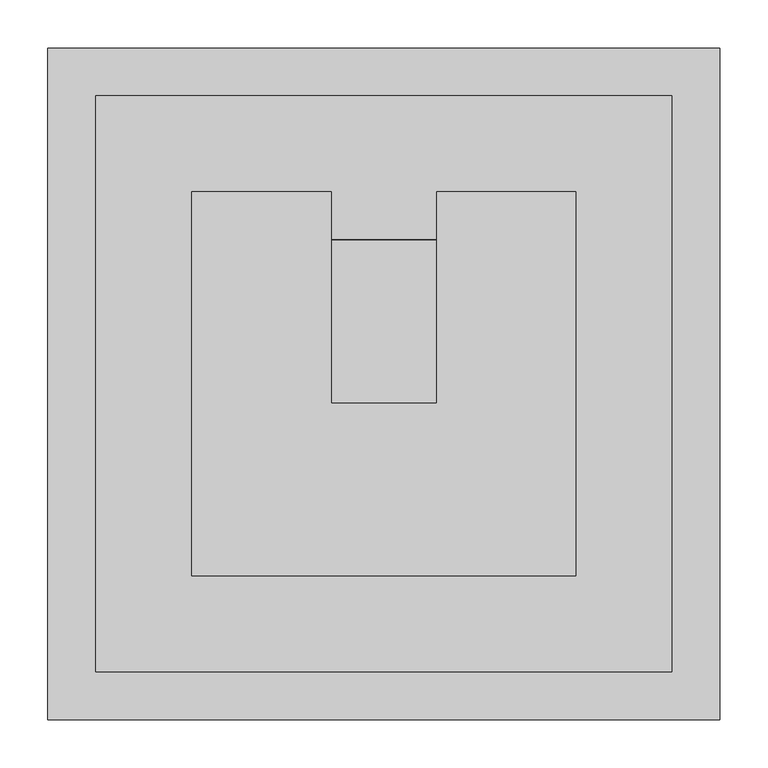
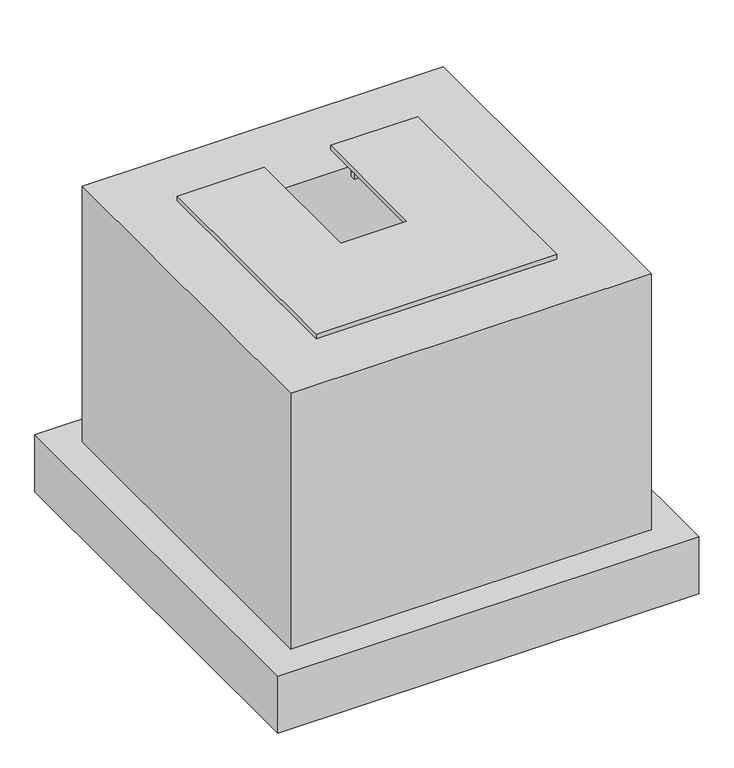
"""IFC4 building model written with IfcOpenShell, lengths in millimetres: proxy geometry, Catchpit : Rainwater Catchpit."""

import ifcopenshell
import ifcopenshell.guid

model = None  # the IFC model being written
_history = None  # IfcOwnerHistory: only IFC2X3 demands one
_inside = {}  # id of a spatial element -> (the spatial element, [elements in it])
_under = {}  # id of a project, library or spatial element -> (it, [spatial elements below it])
_declared = {}  # id of a project -> (the project, [libraries it declares])
_typed = {}  # id of a type object -> (the type object, [elements of that type])
_made_of = {}  # id of a material, layer set ... -> (it, [elements and type objects made of it])


def new_model(schema):
    """Start an empty IFC model of exactly this schema.

    Asked for "IFC4X3", IfcOpenShell would pick the latest addendum, in which some entities
    have other attributes; the version numbers below select the first issue.
    IFC2X3 requires an IfcOwnerHistory on every rooted entity: one is made here for all.
    """
    global model, _history
    if schema == "IFC4X3":
        model = ifcopenshell.file(schema_version=(4, 3, 0, 0))
    else:
        model = ifcopenshell.file(schema=schema)
    _inside.clear()
    _under.clear()
    _declared.clear()
    _typed.clear()
    _made_of.clear()
    _history = None
    if model.schema == "IFC2X3":
        org = make("IfcOrganization", Name="unknown")
        user = make(
            "IfcPersonAndOrganization",
            ThePerson=make("IfcPerson", FamilyName="unknown"),
            TheOrganization=org,
        )
        app = make(
            "IfcApplication",
            ApplicationDeveloper=org,
            Version="unknown",
            ApplicationFullName="unknown",
            ApplicationIdentifier="unknown",
        )
        _history = make(
            "IfcOwnerHistory",
            OwningUser=user,
            OwningApplication=app,
            ChangeAction="ADDED",
            CreationDate=0,
        )
    return model


def make(cls, **values):
    """One entity of the class cls with the attributes given. An attribute that is None is left unset."""
    return model.create_entity(
        cls, **{name: value for name, value in values.items() if value is not None}
    )


def rooted(cls, **values):
    """An entity with a GlobalId (a new one), such as an element, a storey or a relation."""
    return make(cls, GlobalId=ifcopenshell.guid.new(), OwnerHistory=_history, **values)


def si_unit(unit_type, name, prefix=None):
    """IfcSIUnit, for example si_unit("LENGTHUNIT", "METRE", prefix="MILLI")."""
    return make("IfcSIUnit", UnitType=unit_type, Prefix=prefix, Name=name)


def assignment(units):
    """IfcUnitAssignment: the units of a project."""
    return None if units is None else make("IfcUnitAssignment", Units=units)


def point(xyz):
    """IfcCartesianPoint."""
    return None if xyz is None else make("IfcCartesianPoint", Coordinates=xyz)


def direction(xyz):
    """IfcDirection."""
    return None if xyz is None else make("IfcDirection", DirectionRatios=xyz)


def frame(location, z_axis=None, x_axis=None):
    """IfcAxis2Placement3D, a coordinate frame: its origin and axes. An axis left out is left unset."""
    return make(
        "IfcAxis2Placement3D",
        Location=point(location),
        Axis=direction(z_axis),
        RefDirection=direction(x_axis),
    )


def origin():
    """The frame at (0, 0, 0) with its axes left unset."""
    return frame((0.0, 0.0, 0.0))


def origin_with_axes():
    """The frame at (0, 0, 0) with the z axis (0, 0, 1) and the x axis (1, 0, 0) written out."""
    return frame((0.0, 0.0, 0.0), z_axis=(0.0, 0.0, 1.0), x_axis=(1.0, 0.0, 0.0))


def place(relative_to, where):
    """IfcLocalPlacement: puts the frame where relative to a parent placement (None: the world)."""
    return make(
        "IfcLocalPlacement", PlacementRelTo=relative_to, RelativePlacement=where
    )


def context(
    kind, dimensions, precision=None, world=None, true_north=None, identifier=None
):
    """IfcGeometricRepresentationContext, for example the 3D "Model" context."""
    return make(
        "IfcGeometricRepresentationContext",
        ContextIdentifier=identifier,
        ContextType=kind,
        CoordinateSpaceDimension=dimensions,
        Precision=precision,
        WorldCoordinateSystem=world,
        TrueNorth=true_north,
    )


def project(units=None, contexts=None):
    """IfcProject with its units and contexts."""
    return rooted(
        "IfcProject",
        Name="project",
        RepresentationContexts=contexts,
        UnitsInContext=assignment(units),
    )


def spatial(cls, under=None, at=None, **own):
    """A site, building, storey or space (cls), placed at a placement, below another one or the project."""
    s = rooted(cls, ObjectPlacement=at, **own)
    if under is not None:
        _under.setdefault(under.id(), (under, []))[1].append(s)
    return s


def polyline(points):
    """IfcPolyline through the points."""
    return make("IfcPolyline", Points=[point(p) for p in points])


def outline(outer, holes=None, kind="AREA"):
    """IfcArbitraryClosedProfileDef: a profile drawn as a closed curve; with holes, ...WithVoids."""
    if holes is None:
        return make("IfcArbitraryClosedProfileDef", ProfileType=kind, OuterCurve=outer)
    return make(
        "IfcArbitraryProfileDefWithVoids",
        ProfileType=kind,
        OuterCurve=outer,
        InnerCurves=holes,
    )


def extrude(swept, where, along, depth):
    """IfcExtrudedAreaSolid: the profile swept, set in the frame where, extruded along a direction by depth."""
    return make(
        "IfcExtrudedAreaSolid",
        SweptArea=swept,
        Position=where,
        ExtrudedDirection=direction(along),
        Depth=depth,
    )


def faces_of(points, faces, orient=None, outer=None):
    """IfcFace entities. A face is a list of loops; a loop is a list of indices into points, from 0.

    orient and outer hold one flag for each loop. By default every Orientation is true, the
    first loop of a face is its IfcFaceOuterBound and the others are IfcFaceBound.
    """
    made = []
    for i, loops in enumerate(faces):
        bounds = []
        for j, loop in enumerate(loops):
            is_outer = j == 0 if outer is None else outer[i][j]
            bounds.append(
                make(
                    "IfcFaceOuterBound" if is_outer else "IfcFaceBound",
                    Bound=make("IfcPolyLoop", Polygon=[points[k] for k in loop]),
                    Orientation=True if orient is None else orient[i][j],
                )
            )
        made.append(make("IfcFace", Bounds=bounds))
    return made


def faceted_brep(points, faces, orient=None, outer=None, voids=None):
    """IfcFacetedBrep: a solid bounded by flat faces; with voids (closed shells), ...WithVoids."""
    shared = [point(p) for p in points]
    hull = make("IfcClosedShell", CfsFaces=faces_of(shared, faces, orient, outer))
    if voids is None:
        return make("IfcFacetedBrep", Outer=hull)
    return make(
        "IfcFacetedBrepWithVoids",
        Outer=hull,
        Voids=[
            make(cls, CfsFaces=faces_of(shared, fs, o, b)) for cls, fs, o, b in voids
        ],
    )


def shape(context_of_items, identifier, shape_type, items):
    """IfcShapeRepresentation: the items that make up one representation, for example the "Body"."""
    return make(
        "IfcShapeRepresentation",
        ContextOfItems=context_of_items,
        RepresentationIdentifier=identifier,
        RepresentationType=shape_type,
        Items=items,
    )


def source(mapping_origin, context_of_items, identifier, shape_type, items):
    """IfcRepresentationMap: a shape defined once, which mapped items show again and again."""
    return make(
        "IfcRepresentationMap",
        MappingOrigin=mapping_origin,
        MappedRepresentation=shape(context_of_items, identifier, shape_type, items),
    )


def transform(
    local_origin,
    x_axis=None,
    y_axis=None,
    z_axis=None,
    scale=None,
    scale2=None,
    scale3=None,
    uniform=True,
):
    """IfcCartesianTransformationOperator3D, or its non-uniform kind. x_axis, y_axis, z_axis: its Axis1, 2, 3."""
    if uniform:
        return make(
            "IfcCartesianTransformationOperator3D",
            Axis1=direction(x_axis),
            Axis2=direction(y_axis),
            LocalOrigin=point(local_origin),
            Scale=scale,
            Axis3=direction(z_axis),
        )
    return make(
        "IfcCartesianTransformationOperator3DnonUniform",
        Axis1=direction(x_axis),
        Axis2=direction(y_axis),
        LocalOrigin=point(local_origin),
        Scale=scale,
        Axis3=direction(z_axis),
        Scale2=scale2,
        Scale3=scale3,
    )


def mapped(mapping_source, mapping_target):
    """IfcMappedItem: shows the shape of a source again, moved by a transform."""
    return make(
        "IfcMappedItem", MappingSource=mapping_source, MappingTarget=mapping_target
    )


def made_of(thing, what):
    """Note that an element or type object is made of a material, layer set ...; save() writes the relation."""
    if what is not None:
        _made_of.setdefault(what.id(), (what, []))[1].append(thing)
    return thing


def element(
    cls,
    number,
    at=None,
    inside=None,
    cuts=None,
    type_object=None,
    material=None,
    context=None,
    identifier="Body",
    shape_type=None,
    held_by="IfcProductDefinitionShape",
    body=None,
    shapes=None,
    **own,
):
    """One element of the class cls, such as IfcWall. Its Tag is "e" and its number.

    at: its placement. inside: the storey or other place that contains it. cuts: it is an
    opening in that element (IfcRelVoidsElement). A single representation is given by context,
    identifier, shape_type and body (its items); several are given by shapes. held_by: the class
    of the entity that holds the representations. save() writes the other relations.
    """
    e = rooted(cls, Tag="e%d" % number, ObjectPlacement=at, **own)
    if body is not None:
        shapes = [shape(context, identifier, shape_type, body)]
    if shapes is not None:
        e.Representation = make(held_by, Representations=shapes)
    if inside is not None:
        _inside.setdefault(inside.id(), (inside, []))[1].append(e)
    if cuts is not None:
        rooted(
            "IfcRelVoidsElement", RelatingBuildingElement=cuts, RelatedOpeningElement=e
        )
    if type_object is not None:
        _typed.setdefault(type_object.id(), (type_object, []))[1].append(e)
    return made_of(e, material)


def aggregate(whole, parts):
    """IfcRelAggregates: a whole, such as a stair, and the parts it consists of."""
    return rooted("IfcRelAggregates", RelatingObject=whole, RelatedObjects=parts)


def save(model, path):
    """Write the relations noted so far, then the file.

    IfcRelAggregates (storeys below a building ...), IfcRelContainedInSpatialStructure (elements
    in a storey), IfcRelDefinesByType, IfcRelAssociatesMaterial and IfcRelDeclares: one each for
    every whole, place, type object, material and project.
    """
    for whole, parts in _under.values():
        aggregate(whole, parts)
    for where, things in _inside.values():
        rooted(
            "IfcRelContainedInSpatialStructure",
            RelatedElements=things,
            RelatingStructure=where,
        )
    for kind, things in _typed.values():
        rooted("IfcRelDefinesByType", RelatedObjects=things, RelatingType=kind)
    for what, things in _made_of.values():
        rooted("IfcRelAssociatesMaterial", RelatedObjects=things, RelatingMaterial=what)
    for by, libraries in _declared.values():
        rooted("IfcRelDeclares", RelatingContext=by, RelatedDefinitions=libraries)
    model.write(path)


def generic_models_4b8b6a59(model_context):
    return source(origin(), model_context, "Body", "SolidModel", [
        extrude(outline(polyline([(-55.0, 140.0), (-55.0, 132.0), (-132.0, 132.0), (-132.0, -132.0), (132.0, -132.0), (132.0, 132.0), (55.0, 132.0), (55.0, 140.0), (140.0, 140.0), (140.0, -140.0), (-140.0, -140.0), (-140.0, 140.0), (-55.0, 140.0)])), frame((0.0, 0.0, -10.0), z_axis=(0.0, 0.0, 1.0), x_axis=(1.0, 0.0, 0.0)), (0.0, 0.0, 1.0), 10.0),
        extrude(outline(polyline([(-55.0, 200.0), (-55.0, -20.0), (55.0, -20.0), (55.0, 200.0), (200.0, 200.0), (200.0, -200.0), (-200.0, -200.0), (-200.0, 200.0), (-55.0, 200.0)])), origin_with_axes(), (0.0, 0.0, 1.0), 8.0),
        faceted_brep([(150.0, -150.0, -300.0), (150.0, 150.0, -300.0), (-150.0, 150.0, -300.0), (-150.0, -150.0, -300.0), (300.0, 300.0, -450.0), (300.0, -300.0, -450.0), (-300.0, -300.0, -450.0), (-300.0, 300.0, -450.0), (-300.0, 300.0, 0.0), (300.0, 300.0, 0.0), (-300.0, -300.0, 0.0), (300.0, -300.0, 0.0), (150.0, 150.0, 0.0), (150.0, -150.0, 0.0), (-150.0, -150.0, 0.0), (-150.0, 150.0, 0.0)], [[[0, 1, 2, 3]], [[4, 5, 6, 7]], [[4, 7, 8, 9]], [[8, 7, 6, 10]], [[10, 6, 5, 11]], [[11, 5, 4, 9]], [[9, 8, 10, 11], [12, 13, 14, 15]], [[13, 12, 1, 0]], [[14, 13, 0, 3]], [[15, 14, 3, 2]], [[12, 15, 2, 1]]]),
        extrude(outline(polyline([(350.0, 350.0), (350.0, -350.0), (-350.0, -350.0), (-350.0, 350.0), (350.0, 350.0)])), frame((0.0, 0.0, -550.0), z_axis=(0.0, 0.0, 1.0), x_axis=(1.0, 0.0, 0.0)), (0.0, 0.0, 1.0), 100.0),
    ])


if __name__ == "__main__":
    model = new_model("IFC4")
    model_context = context("Model", 3, world=origin())
    ifc_project = project(units=[si_unit("LENGTHUNIT", "METRE", prefix="MILLI")], contexts=[model_context])
    site = spatial("IfcSite", under=ifc_project)
    building = spatial("IfcBuilding", under=site)
    placement = place(None, origin())
    generic_models_shape = generic_models_4b8b6a59(model_context)
    element("IfcBuildingElementProxy", 1, Name="Catchpit : Rainwater Catchpit", ObjectType="Catchpit : Rainwater Catchpit", at=placement, inside=building, context=model_context, shape_type="MappedRepresentation", body=[
        mapped(generic_models_shape, transform((0.0, 0.0, 0.0), x_axis=(1.0, 0.0, 0.0), y_axis=(0.0, 1.0, 0.0), z_axis=(0.0, 0.0, 1.0))),
    ])
    save(model, "model.ifc")

# Revit data of these elements
# Type "Catchpit : Rainwater Catchpit"
#   Width = 300 mm
#   Wall Thk = 150 mm
#   Slab Thk = 150 mm
#   Length = 300 mm
#   Lean Thk = 100 mm
#   Lean Edge = 50 mm
#   Height = 300 mm
#   FB Thk = 8 mm
#   FB Length = 10 mm
#   Cutting Width = 110 mm
#   Cutting Length = 220 mm
#   Chk'd PL Thk = 8 mm
#   Structure Material = none
#   Lean_Material = none
#   CHK`D = none
#   Default Elevation = 0
